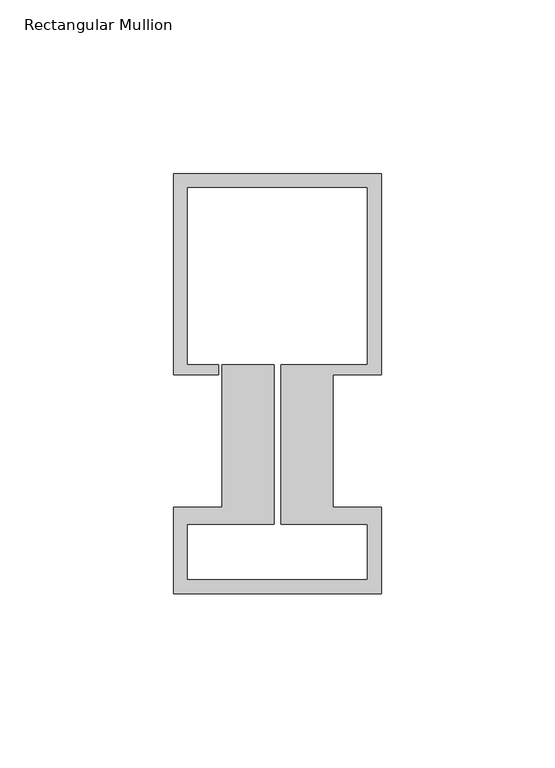
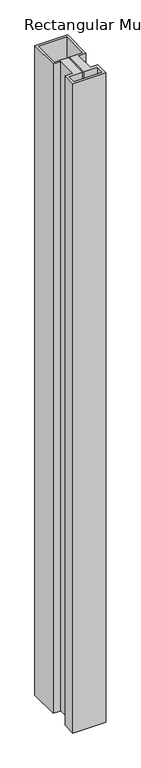
"""IFC4 building model written with IfcOpenShell, lengths in millimetres: member geometry, Rectangular Mullion : Schueco_FWS-60-SI_Tran_CovCap-20mm_Tran-55mm."""

from ifc_helpers import new_model, si_unit, frame, origin, place, context, project, spatial, polyline, outline, extrude, source, transform, mapped, element, save


def rectangular_mullion_fb91133a(model_context):
    return source(origin(), model_context, "Body", "SweptSolid", [
        extrude(outline(polyline([(0.0, 96.0), (0.0, 38.0), (-14.0, 38.0), (-14.0, -0.1), (0.0, -0.1), (0.0, -25.0), (-60.0, -25.0), (-60.0, -0.1), (-46.0, -0.1), (-46.0, 41.0), (-31.0, 41.0), (-31.0, -5.0), (-56.0, -5.0), (-56.0, -21.0), (-4.0, -21.0), (-4.0, -5.0), (-29.0, -5.0), (-29.0, 41.0), (-4.0, 41.0), (-4.0, 92.0), (-56.0, 92.0), (-56.0, 41.0), (-47.0, 41.0), (-47.0, 38.0), (-60.0, 38.0), (-60.0, 96.0), (0.0, 96.0)])), frame((0.0, 0.0, -1260.0), z_axis=(0.0, 0.0, 1.0), x_axis=(1.0, 0.0, 0.0)), (0.0, 0.0, 1.0), 1260.0),
    ])


if __name__ == "__main__":
    model = new_model("IFC4")
    model_context = context("Model", 3, world=origin())
    ifc_project = project(units=[si_unit("LENGTHUNIT", "METRE", prefix="MILLI")], contexts=[model_context])
    site = spatial("IfcSite", under=ifc_project)
    building = spatial("IfcBuilding", under=site)
    placement = place(None, origin())
    rectangular_mullion_shape = rectangular_mullion_fb91133a(model_context)
    element("IfcMember", 1, ObjectType="Rectangular Mullion : Schueco_FWS-60-SI_Tran_CovCap-20mm_Tran-55mm", at=placement, inside=building, context=model_context, shape_type="MappedRepresentation", body=[
        mapped(rectangular_mullion_shape, transform((0.0, 0.0, 0.0), x_axis=(1.0, 0.0, 0.0), y_axis=(0.0, 1.0, 0.0), z_axis=(0.0, 0.0, 1.0))),
    ])
    save(model, "model.ifc")

# Revit data of these elements
# Type "Rectangular Mullion : Schueco_FWS-60-SI_Tran_CovCap-20mm_Tran-55mm"
#   Model = "FWS 60.SI"
#   Manufacturer = "Schueco International KG"
#   Type Comments = "Transom"
#   Schueco thermal insulation standard = "Suitable for passive houses"
#   Burglar resistance = "RC 3"
#   Thermal insulation = "to 0.70 W/(m²K)"
#   built-in parameter 1007322 = 0.396982 (stored number, unit not read)
#   built-in parameter 1007321 = 0.0524934 (stored number, unit not read)
#   built-in parameter 1007320 = 0.0524934 (stored number, unit not read)
# Element 1 (IfcMember, "Rectangular Mullion : Schueco_FWS-60-SI_Tran_CovCap-20mm_Tran-55mm")
#   Materials on its faces: "Alu"
# Materials
#   "Alu": class "Glas", colour RGB 140 140 140, transparency 0
